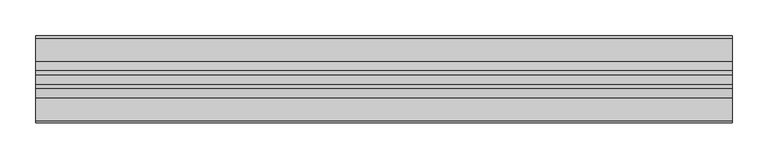
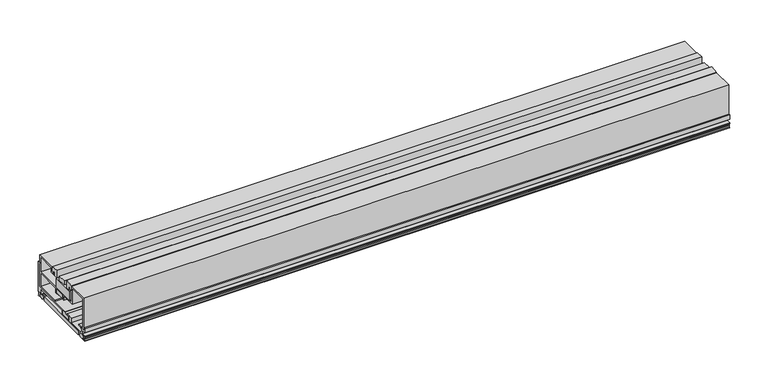
"""IFC4 building model written with IfcOpenShell, lengths in millimetres: proxy geometry, Generic Models 3:Generic Models 1:2:Generic Models 1:2 : Generic Models 3:Generic Models 1:300625:328150:Generic Models 1:2:Generic Models 1:2 : Generic Models 3:Generic Models 1:300625:328150 : Generic Models 3:Generic Models 1:2:Generic Models 1:2 : Generic Models 3:Generic Models 1:300625:328150:1 : Generic Models 3:Generic Models 1:2:Generic Models 1:2 : Generic Models 3:Generic Models 1:300625:328150:Generic Models 1:2:Generic Models 1:2 : Generic Models 3:Generic Models 1:300625:328150 : Generic Models 3:Generic Models 1:2:Generic Models 1:2 : Generic Models 3:Generic Models 1:300625:328150:300962."""

from ifc_helpers import new_model, si_unit, frame, origin, origin_with_axes, place, context, project, spatial, polyline, outline, extrude, source, transform, mapped, element, save


def generic_models_5bfda5a7(model_context):
    return source(origin(), model_context, "Body", "SweptSolid", [
        extrude(outline(polyline([(570371.6742239, -579015.3141007), (570371.6742239, -579104.2141007), (569476.3242239, -579104.2141007), (569476.3242239, -579015.3141007), (570371.6742239, -579015.3141007)])), origin_with_axes(), (0.0, 0.0, 1.0), 6.35),
        extrude(outline(polyline([(-579000.519923, 5.3842368), (-579000.8336091, 3.175), (-579000.519923, 0.9657632), (-579000.1425144, 0.0), (-579006.0106065, 0.0), (-579005.1503256, 0.3863176), (-579003.8407504, 1.469803), (-579003.2403969, 2.8200508), (-579003.4431848, 4.2258271), (-579004.4173898, 5.4672112), (-579006.0106065, 6.35), (-579000.1425144, 6.35), (-579000.519923, 5.3842368)])), frame((569476.3242239, 0.0, 0.0), z_axis=(1.0, 0.0, 0.0), x_axis=(0.0, 1.0, 0.0)), (0.0, 0.0, 1.0), 895.35),
        extrude(outline(polyline([(-579004.0833699, 1.7974191), (-579005.4048639, 0.692685), (-579007.3144782, 0.0796039), (-579008.3742341, 0.0), (-579009.4339901, 0.0796039), (-579011.3436043, 0.692685), (-579012.6650983, 1.7974191), (-579013.1367341, 3.175), (-579012.6650983, 4.5525809), (-579011.3436043, 5.657315), (-579009.4339901, 6.2703961), (-579008.3742341, 6.35), (-579007.3144782, 6.2703961), (-579005.4048639, 5.657315), (-579004.0833699, 4.5525809), (-579003.6117341, 3.175), (-579004.0833699, 1.7974191)])), frame((569476.3242239, 0.0, 0.0), z_axis=(1.0, 0.0, 0.0), x_axis=(0.0, 1.0, 0.0)), (0.0, 0.0, 1.0), 895.35),
        extrude(outline(polyline([(-579111.68681, 0.0796039), (-579112.746566, 0.0), (-579113.8063219, 0.0796039), (-579115.7159362, 0.692685), (-579117.0374302, 1.7974191), (-579117.509066, 3.175), (-579117.0374302, 4.5525809), (-579115.7159362, 5.657315), (-579113.8063219, 6.2703961), (-579112.746566, 6.35), (-579111.68681, 6.2703961), (-579109.7771958, 5.657315), (-579108.4557018, 4.5525809), (-579107.984066, 3.175), (-579108.4557018, 1.7974191), (-579109.7771958, 0.692685), (-579111.68681, 0.0796039)])), frame((569476.3242239, 0.0, 0.0), z_axis=(1.0, 0.0, 0.0), x_axis=(0.0, 1.0, 0.0)), (0.0, 0.0, 1.0), 969.9625),
        extrude(outline(polyline([(-579115.1101936, 0.0), (-579120.9782857, 0.0), (-579120.6008771, 0.9657632), (-579120.287191, 3.175), (-579120.6008771, 5.3842368), (-579120.9782857, 6.35), (-579115.1101936, 6.35), (-579116.7034103, 5.4672112), (-579117.6776153, 4.2258271), (-579117.8804032, 2.8200508), (-579117.2800497, 1.469803), (-579115.9704745, 0.3863176), (-579115.1101936, 0.0)])), frame((569476.3242239, 0.0, 0.0), z_axis=(1.0, 0.0, 0.0), x_axis=(0.0, 1.0, 0.0)), (0.0, 0.0, 1.0), 969.9625),
        extrude(outline(polyline([(570446.2867239, -579047.2017564), (570446.2867239, -579080.4885915), (569476.3242239, -579080.4885915), (569476.3242239, -579047.2017564), (570446.2867239, -579047.2017564)])), frame((0.0, 0.0, 40.9290939), z_axis=(0.0, 0.0, 1.0), x_axis=(1.0, 0.0, 0.0)), (0.0, 0.0, 1.0), 14.2115027),
        extrude(outline(polyline([(570446.2867239, -579063.676291), (570446.2867239, -579079.7877272), (569476.3242239, -579079.7877272), (569476.3242239, -579063.676291), (570446.2867239, -579063.676291)])), frame((0.0, 0.0, 8.0979388), z_axis=(0.0, 0.0, 1.0), x_axis=(1.0, 0.0, 0.0)), (0.0, 0.0, 1.0), 6.0797872),
        extrude(outline(polyline([(-579003.1775737, 53.9246391), (-579000.1425144, 53.9246391), (-579000.1425144, 6.35), (-579008.035108, 6.35), (-579008.035108, 13.721742), (-579062.0043495, 13.721742), (-579062.0043495, 6.35), (-579068.5401208, 6.35), (-579068.5401208, 8.0979388), (-579063.676291, 8.0979388), (-579063.676291, 14.1777261), (-579068.5401208, 14.1777261), (-579068.5401208, 15.4696809), (-579001.8904532, 15.4696809), (-579001.8904532, 52.2575319), (-579003.1775737, 52.2575319), (-579003.1775737, 53.9246391)])), frame((569476.3242239, 0.0, 0.0), z_axis=(1.0, 0.0, 0.0), x_axis=(0.0, 1.0, 0.0)), (0.0, 0.0, 1.0), 969.9625),
        extrude(outline(polyline([(-579085.6315392, 8.0979388), (-579085.6315392, 15.4696809), (-579074.9238974, 15.4696809), (-579074.9238974, 14.1777261), (-579079.7877272, 14.1777261), (-579079.7877272, 8.0979388), (-579074.9238974, 8.0979388), (-579074.9238974, 6.35), (-579120.9782857, 6.35), (-579120.9782857, 8.0979388), (-579114.5945091, 8.0979388), (-579114.5945091, 13.721742), (-579120.9782857, 13.721742), (-579120.9782857, 20.2285817), (-579119.1114916, 20.2285817), (-579119.1114916, 15.4696809), (-579110.1654191, 15.4696809), (-579110.1654191, 14.5730392), (-579112.5861229, 13.9244136), (-579111.6757362, 8.0979388), (-579085.6315392, 8.0979388)])), frame((569476.3242239, 0.0, 0.0), z_axis=(1.0, 0.0, 0.0), x_axis=(0.0, 1.0, 0.0)), (0.0, 0.0, 1.0), 969.9625),
        extrude(outline(polyline([(570446.2867239, -579047.8857325), (570446.2867239, -579063.9971687), (569476.3242239, -579063.9971687), (569476.3242239, -579047.8857325), (570446.2867239, -579047.8857325)])), frame((0.0, 0.0, 32.9493731), z_axis=(0.0, 0.0, 1.0), x_axis=(1.0, 0.0, 0.0)), (0.0, 0.0, 1.0), 6.0797872),
        extrude(outline(polyline([(570446.2867239, -579054.6832724), (570446.2867239, -579067.3832724), (569476.3242239, -579067.3832724), (569476.3242239, -579054.6832724), (570446.2867239, -579054.6832724)])), frame((0.0, 0.0, 57.1165274), z_axis=(0.0, 0.0, 1.0), x_axis=(1.0, 0.0, 0.0)), (0.0, 0.0, 1.0), 6.3435484),
        extrude(outline(polyline([(-579078.8757591, 62.433193), (-579081.7214373, 62.433193), (-579081.7214373, 59.4893332), (-579086.0195091, 59.4893332), (-579086.0195091, 67.3290426), (-579074.1217032, 68.7899095), (-579074.1217032, 56.7196524), (-579078.8757591, 56.7196524), (-579078.8757591, 62.433193)])), frame((569476.3242239, 0.0, 0.0), z_axis=(1.0, 0.0, 0.0), x_axis=(0.0, 1.0, 0.0)), (0.0, 0.0, 1.0), 969.9625),
        extrude(outline(polyline([(-579036.0470357, 67.3290426), (-579036.0470357, 59.4893332), (-579040.3451075, 59.4893332), (-579040.3451075, 62.433193), (-579043.1907857, 62.433193), (-579043.1907857, 56.7196524), (-579047.9448415, 56.7196524), (-579047.9448415, 68.7899095), (-579036.0470357, 67.3290426)])), frame((569476.3242239, 0.0, 0.0), z_axis=(1.0, 0.0, 0.0), x_axis=(0.0, 1.0, 0.0)), (0.0, 0.0, 1.0), 969.9625),
        extrude(outline(polyline([(-579118.1663841, 15.5459822), (-579118.1663841, 66.3122056), (-579086.4163841, 66.3122056), (-579086.4163841, 59.0924582), (-579081.3245623, 59.0924582), (-579081.3245623, 62.036318), (-579079.2726341, 62.036318), (-579079.2726341, 57.1165274), (-579086.4163841, 57.1165274), (-579086.4163841, 40.9290939), (-579059.1333389, 40.9290939), (-579059.1333389, 39.0291604), (-579063.9971687, 39.0291604), (-579063.9971687, 32.9493731), (-579059.1333389, 32.9493731), (-579059.1333389, 31.6574183), (-579065.8971022, 31.6574183), (-579065.8971022, 39.0291604), (-579088.3163176, 39.0291604), (-579088.3163176, 64.4122721), (-579115.6584719, 64.4122721), (-579115.6584719, 17.4459157), (-579105.079253, 17.4459157), (-579105.079253, 15.5459822), (-579118.1663841, 15.5459822)])), frame((569476.3242239, 0.0, 0.0), z_axis=(1.0, 0.0, 0.0), x_axis=(0.0, 1.0, 0.0)), (0.0, 0.0, 1.0), 969.9625),
        extrude(outline(polyline([(-579040.7419825, 62.036318), (-579040.7419825, 59.0924582), (-579035.6501607, 59.0924582), (-579035.6501607, 66.3122056), (-579003.8663841, 66.3122056), (-579003.8663841, 15.5459822), (-579042.7939107, 15.5459822), (-579042.7939107, 17.4681948), (-579005.8423149, 17.4681948), (-579005.8423149, 39.0291604), (-579045.985799, 39.0291604), (-579045.985799, 31.6574183), (-579052.7495623, 31.6574183), (-579052.7495623, 32.9493731), (-579047.8857325, 32.9493731), (-579047.8857325, 39.0291604), (-579052.7495623, 39.0291604), (-579052.7495623, 40.9290939), (-579005.8423149, 40.9290939), (-579005.8423149, 64.4024065), (-579033.7502272, 64.4024065), (-579033.7502272, 57.1165274), (-579042.7939107, 57.1165274), (-579042.7939107, 62.036318), (-579040.7419825, 62.036318)])), frame((569476.3242239, 0.0, 0.0), z_axis=(1.0, 0.0, 0.0), x_axis=(0.0, 1.0, 0.0)), (0.0, 0.0, 1.0), 969.9625),
    ])


if __name__ == "__main__":
    model = new_model("IFC4")
    model_context = context("Model", 3, world=origin())
    ifc_project = project(units=[si_unit("LENGTHUNIT", "METRE", prefix="MILLI")], contexts=[model_context])
    site = spatial("IfcSite", under=ifc_project)
    building = spatial("IfcBuilding", under=site)
    placement = place(None, origin())
    generic_models_shape = generic_models_5bfda5a7(model_context)
    element("IfcBuildingElementProxy", 1, Name="Generic Models 3:Generic Models 1:2:Generic Models 1:2 : Generic Models 3:Generic Models 1:300625:328150:Generic Models 1:2:Generic Models 1:2 : Generic Models 3:Generic Models 1:300625:328150 : Generic Models 3:Generic Models 1:2:Generic Models 1:2 : Generic Models 3:Generic Models 1:300625:328150:1 : Generic Models 3:Generic Models 1:2:Generic Models 1:2 : Generic Models 3:Generic Models 1:300625:328150:Generic Models 1:2:Generic Models 1:2 : Generic Models 3:Generic Models 1:300625:328150 : Generic Models 3:Generic Models 1:2:Generic Models 1:2 : Generic Models 3:Generic Models 1:300625:328150:300962", ObjectType="Generic Models 3:Generic Models 1:2:Generic Models 1:2 : Generic Models 3:Generic Models 1:300625:328150:Generic Models 1:2:Generic Models 1:2 : Generic Models 3:Generic Models 1:300625:328150 : Generic Models 3:Generic Models 1:2:Generic Models 1:2 : Generic Models 3:Generic Models 1:300625:328150:1 : Generic Models 3:Generic Models 1:2:Generic Models 1:2 : Generic Models 3:Generic Models 1:300625:328150:Generic Models 1:2:Generic Models 1:2 : Generic Models 3:Generic Models 1:300625:328150 : Generic Models 3:Generic Models 1:2:Generic Models 1:2 : Generic Models 3:Generic Models 1:300625:328150:300962", at=placement, inside=building, context=model_context, shape_type="MappedRepresentation", body=[
        mapped(generic_models_shape, transform((0.0, 0.0, 0.0), x_axis=(1.0, 0.0, 0.0), y_axis=(0.0, 1.0, 0.0), z_axis=(0.0, 0.0, 1.0))),
    ])
    save(model, "model.ifc")

# Revit data of these elements
# Type "Generic Models 3:Generic Models 1:2:Generic Models 1:2 : Generic Models 3:Generic Models 1:300625:328150:Generic Models 1:2:Generic Models 1:2 : Generic Models 3:Generic Models 1:300625:328150 : Generic Models 3:Generic Models 1:2:Generic Models 1:2 : Generic Models 3:Generic Models 1:300625:328150:1 : Generic Models 3:Generic Models 1:2:Generic Models 1:2 : Generic Models 3:Generic Models 1:300625:328150:Generic Models 1:2:Generic Models 1:2 : Generic Models 3:Generic Models 1:300625:328150 : Generic Models 3:Generic Models 1:2:Generic Models 1:2 : Generic Models 3:Generic Models 1:300625:328150:300962"
#   NameOverride = "Generic Models 3:Generic Models 1:2:Generic Models 1:2 : Generic Models 3:Generic Models 1:300625:328150:Generic Models 1:2:Generic Models 1:2 : Generic Models 3:Generic Models 1:300625:328150 : Generic Models 3:Generic Models 1:2:Generic Models 1:2 : Generic Models 3:Generic Models 1:300625:328150:300962"
#   ObjectTypeOverride = "Generic Models 1:2:Generic Models 1:2 : Generic Models 3:Generic Models 1:300625:328150 : Generic Models 3:Generic Models 1:2:Generic Models 1:2 : Generic Models 3:Generic Models 1:300625:328150"
#   Reference = "Generic Models 1"
#   Tag = "300962"
# Element 1 (IfcBuildingElementProxy, "Generic Models 3:Generic Models 1:2:Generic Models 1:2 : Generic Models 3:Generic Models 1:300625:328150:Generic Models 1:2:Generic Models 1:2 : Generic Models 3:Generic Models 1:300625:328150 : Generic Models 3:Generic Models 1:2:Generic Models 1:2 : Generic Models 3:Generic Models 1:300625:328150:1 : Generic Models 3:Generic Models 1:2:Generic Models 1:2 : Generic Models 3:Generic Models 1:300625:328150:Generic Models 1:2:Generic Models 1:2 : Generic Models 3:Generic Models 1:300625:328150 : Generic Models 3:Generic Models 1:2:Generic Models 1:2 : Generic Models 3:Generic Models 1:300625:328150:300962")
#   Materials on its faces: "THERMAL BROKEN ALUMINUM STOREFRONT", "SEALANT & BACKER ROD", "Compression Gasket_1", "Shim_1", "Desiccant Sealant_1"
# Materials
#   "THERMAL BROKEN ALUMINUM STOREFRONT": class "Unassigned", colour RGB 244 244 244, transparency 0, Cost = 0
#   "SEALANT & BACKER ROD": class "Unassigned", colour RGB 120 120 120, transparency 0, Cost = 0
#   "Compression Gasket_1": class "Unassigned", colour RGB 178 178 178, transparency 0
#   "Shim_1": class "Unassigned", colour RGB 218 218 218, transparency 0
#   "Desiccant Sealant_1": class "Unassigned", colour RGB 120 120 120, transparency 0
